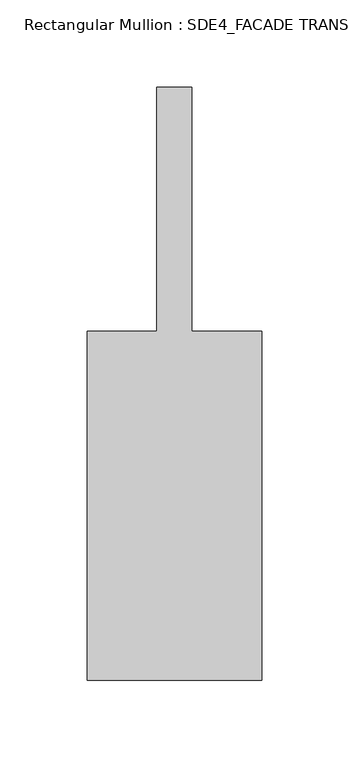
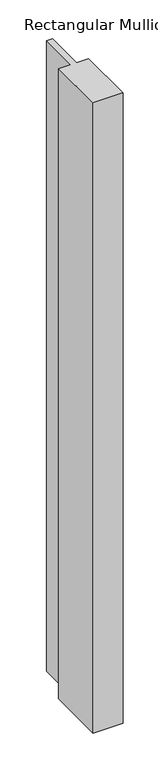
"""IFC4 building model written with IfcOpenShell, lengths in millimetres: member geometry, Rectangular Mullion : SDE4_FACADE TRANSOM TYPE 1."""

from ifc_helpers import new_model, si_unit, frame, origin, place, context, project, spatial, polyline, outline, extrude, source, transform, mapped, element, save


def rectangular_mullion_sde4_facade_transom_type_1_53e51689(model_context):
    return source(origin(), model_context, "Body", "SweptSolid", [
        extrude(outline(polyline([(50.0, -132.5), (-50.0, -132.5), (-50.0, 67.5), (-10.0, 67.5), (-10.0, 207.5), (10.0, 207.5), (10.0, 67.5), (50.0, 67.5), (50.0, -132.5)])), frame((0.0, 0.0, -2239.0), z_axis=(0.0, 0.0, 1.0), x_axis=(1.0, 0.0, 0.0)), (0.0, 0.0, 1.0), 2239.0),
    ])


if __name__ == "__main__":
    model = new_model("IFC4")
    model_context = context("Model", 3, world=origin())
    ifc_project = project(units=[si_unit("LENGTHUNIT", "METRE", prefix="MILLI")], contexts=[model_context])
    site = spatial("IfcSite", under=ifc_project)
    building = spatial("IfcBuilding", under=site)
    placement = place(None, origin())
    rectangular_mullion_sde4_facade_transom_type_1_shape = rectangular_mullion_sde4_facade_transom_type_1_53e51689(model_context)
    element("IfcMember", 1, ObjectType="Rectangular Mullion : SDE4_FACADE TRANSOM TYPE 1", at=placement, inside=building, context=model_context, shape_type="MappedRepresentation", body=[
        mapped(rectangular_mullion_sde4_facade_transom_type_1_shape, transform((0.0, 0.0, 0.0), x_axis=(1.0, 0.0, 0.0), y_axis=(0.0, 1.0, 0.0), z_axis=(0.0, 0.0, 1.0))),
    ])
    save(model, "model.ifc")

# Revit data of these elements
# Type "Rectangular Mullion : SDE4_FACADE TRANSOM TYPE 1"
#   built-in parameter 1007322 = 1.11549 (stored number, unit not read)
#   built-in parameter 1007321 = 0.164042 (stored number, unit not read)
#   built-in parameter 1007320 = 0.164042 (stored number, unit not read)
